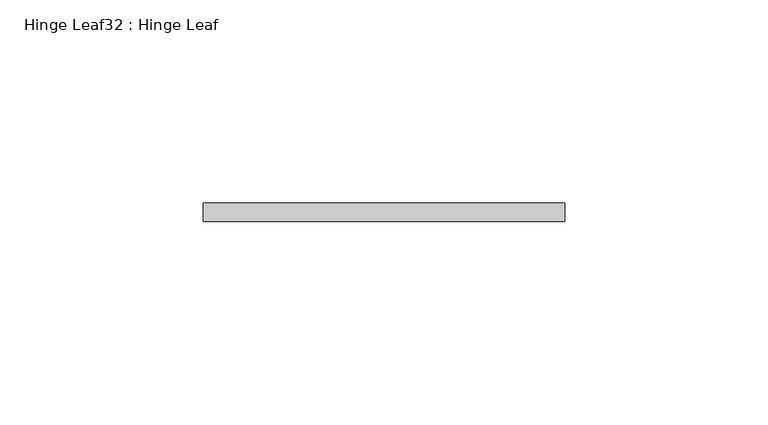
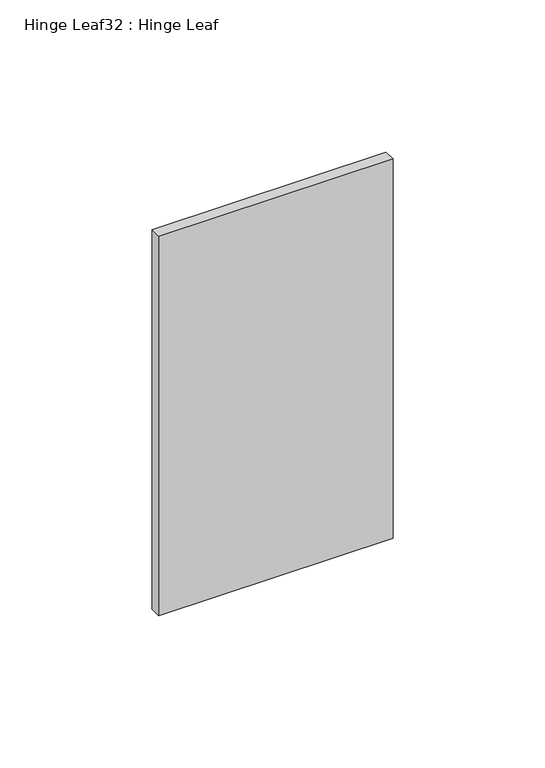
"""IFC4 building model written with IfcOpenShell, lengths in millimetres: proxy geometry, Hinge Leaf32 : Hinge Leaf."""

from ifc_helpers import new_model, si_unit, frame, origin, place, context, project, spatial, polyline, outline, extrude, source, transform, mapped, element, save


def hinge_leaf32_hinge_leaf_bcfbb292(model_context):
    return source(origin(), model_context, "Body", "SweptSolid", [
        extrude(outline(polyline([(587327.7934739, -533980.5883841), (587327.7934739, -533976.0163841), (587416.6934739, -533976.0163841), (587416.6934739, -533980.5883841), (587327.7934739, -533980.5883841)])), frame((0.0, 0.0, 311.15), z_axis=(0.0, 0.0, 1.0), x_axis=(1.0, 0.0, 0.0)), (0.0, 0.0, 1.0), 152.4),
    ])


if __name__ == "__main__":
    model = new_model("IFC4")
    model_context = context("Model", 3, world=origin())
    ifc_project = project(units=[si_unit("LENGTHUNIT", "METRE", prefix="MILLI")], contexts=[model_context])
    site = spatial("IfcSite", under=ifc_project)
    building = spatial("IfcBuilding", under=site)
    placement = place(None, origin())
    hinge_leaf32_hinge_leaf_shape = hinge_leaf32_hinge_leaf_bcfbb292(model_context)
    element("IfcBuildingElementProxy", 1, Name="Hinge Leaf32 : Hinge Leaf", ObjectType="Hinge Leaf32 : Hinge Leaf", at=placement, inside=building, context=model_context, shape_type="MappedRepresentation", body=[
        mapped(hinge_leaf32_hinge_leaf_shape, transform((0.0, 0.0, 0.0), x_axis=(1.0, 0.0, 0.0), y_axis=(0.0, 1.0, 0.0), z_axis=(0.0, 0.0, 1.0))),
    ])
    save(model, "model.ifc")

# Revit data of these elements
# Element 1 (IfcBuildingElementProxy, "Hinge Leaf32 : Hinge Leaf")
#   Materials on its faces: "6\"X6\" WELD-ON STL BUTT HINGE"
# Materials
#   "6\"X6\" WELD-ON STL BUTT HINGE": class "Metal", colour RGB 189 187 185, transparency 0, Description = "Carbon steel", Cost = 0
